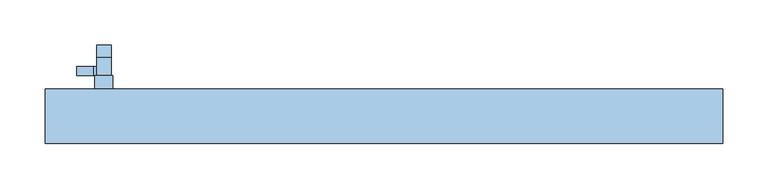
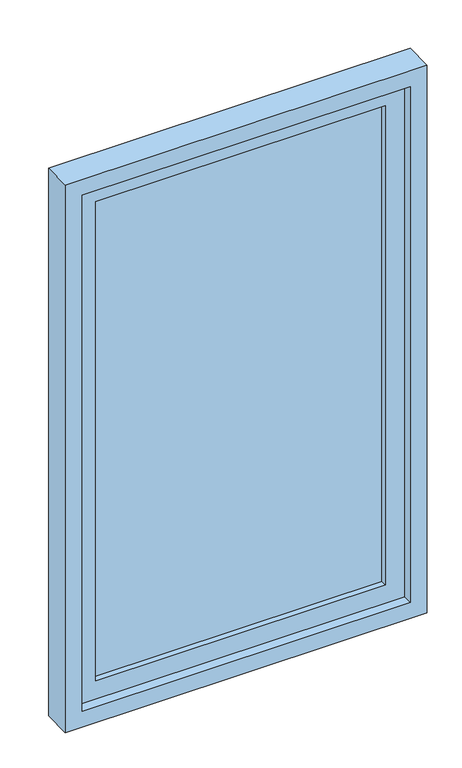
"""IFC4 building model written with IfcOpenShell, lengths in millimetres: window geometry, Inclinar e virar janela - 1 Painel : Inclinar e virar janela - 1 Painel 0,75m."""

from ifc_helpers import new_model, si_unit, point, frame, frame_2d, origin, place, context, project, spatial, polyline, circle_curve, trimmed, segment, composite_curve, outline, extrude, source, transform, mapped, element, save


def window_521f4ff6(model_context):
    return source(origin(), model_context, "Body", "SweptSolid", [
        extrude(outline(composite_curve([segment(polyline([(95.0, 1259.0), (85.0, 1259.0), (85.0, 1277.0), (105.0, 1277.0)]), True, "CONTINUOUS"), segment(trimmed(circle_curve(frame_2d((105.0, 1263.0)), 14.0), [point((105.0, 1277.0))], [point((119.0, 1263.0))], False, "CARTESIAN"), True, "CONTINUOUS"), segment(polyline([(119.0, 1263.0), (119.0, 1120.0), (114.0, 1120.0), (106.9888756, 1235.3294081)]), True, "CONTINUOUS"), segment(trimmed(circle_curve(frame_2d((100.9630874, 1234.9630874)), 6.0369126), [point((106.9888756, 1235.3294081))], [point((100.9630874, 1241.0))], True, "CARTESIAN"), True, "CONTINUOUS"), segment(polyline([(100.9630874, 1241.0), (95.0, 1241.0), (95.0, 1259.0)]), True, "CONTINUOUS")], self_intersect=False)), frame((-318.0, 0.0, 0.0), z_axis=(1.0, 0.0, 0.0), x_axis=(0.0, 1.0, 0.0)), (0.0, 0.0, 1.0), 16.0),
        extrude(outline(polyline([(1259.0, -302.0), (1259.0, -321.9864015), (1257.0348924, -340.0), (1243.0157191, -340.0), (1241.0, -321.9864015), (1241.0, -302.0), (1259.0, -302.0)])), frame((0.0, 85.0, 0.0), z_axis=(0.0, 1.0, 0.0), x_axis=(0.0, 0.0, 1.0)), (0.0, 0.0, 1.0), 10.0),
        extrude(outline(polyline([(-320.0, 85.0), (-300.0, 85.0), (-300.0, 70.0), (-320.0, 70.0), (-320.0, 85.0)])), frame((0.0, 0.0, 1218.0), z_axis=(0.0, 0.0, 1.0), x_axis=(1.0, 0.0, 0.0)), (0.0, 0.0, 1.0), 64.0),
        extrude(outline(polyline([(300.0, 43.0), (-300.0, 43.0), (-300.0, 57.0), (300.0, 57.0), (300.0, 43.0)])), frame((0.0, 0.0, 725.0), z_axis=(0.0, 0.0, 1.0), x_axis=(1.0, 0.0, 0.0)), (0.0, 0.0, 1.0), 1050.0),
        extrude(outline(polyline([(1815.0, -340.0), (685.0, -340.0), (685.0, 340.0), (1815.0, 340.0), (1815.0, -340.0)]), holes=[polyline([(725.0, -300.0), (1775.0, -300.0), (1775.0, 300.0), (725.0, 300.0), (725.0, -300.0)])]), frame((0.0, 30.0, 0.0), z_axis=(0.0, 1.0, 0.0), x_axis=(0.0, 0.0, 1.0)), (0.0, 0.0, 1.0), 40.0),
        extrude(outline(polyline([(1850.0, -375.0), (650.0, -375.0), (650.0, 375.0), (1850.0, 375.0), (1850.0, -375.0)]), holes=[polyline([(685.0, -340.0), (1815.0, -340.0), (1815.0, 340.0), (685.0, 340.0), (685.0, -340.0)])]), frame((0.0, 10.0, 0.0), z_axis=(0.0, 1.0, 0.0), x_axis=(0.0, 0.0, 1.0)), (0.0, 0.0, 1.0), 60.0),
    ])


if __name__ == "__main__":
    model = new_model("IFC4")
    model_context = context("Model", 3, world=origin())
    ifc_project = project(units=[si_unit("LENGTHUNIT", "METRE", prefix="MILLI")], contexts=[model_context])
    site = spatial("IfcSite", under=ifc_project)
    building = spatial("IfcBuilding", under=site)
    placement = place(None, origin())
    window_shape = window_521f4ff6(model_context)
    element("IfcWindow", 1, ObjectType="Inclinar e virar janela - 1 Painel : Inclinar e virar janela - 1 Painel 0,75m", at=placement, inside=building, context=model_context, shape_type="MappedRepresentation", body=[
        mapped(window_shape, transform((0.0, 0.0, 0.0), x_axis=(1.0, 0.0, 0.0), y_axis=(0.0, 1.0, 0.0), z_axis=(0.0, 0.0, 1.0))),
    ])
    save(model, "model.ifc")

# Revit data of these elements
# Type "Inclinar e virar janela - 1 Painel : Inclinar e virar janela - 1 Painel 0,75m"
#   Type Mark = "EF30"
#   Construction Type Id = "SGL"
#   Analytic Construction = "Janelas grandes envidraçadas únicas"
#   W1 = 0.680 m
#   Visual Light Transmittance = 0.9
#   Solar Heat Gain Coefficient = 0.86
#   Rough Width = 0.750 m
#   Rough Height = 1.200 m
#   Largura da moldura do painel = 0.040 m
#   Espessura da moldura do painel = 0.040 m
#   Height = 1.200 m
#   Heat Transfer Coefficient (U) = 5.5617 W/(m²·K)
#   H1 = 1.130 m
#   Largura da estrutura = 0.035 m
#   Espessura da moldura = 0.060 m
#   Altura-padrão do peitoril = 0.650 m
#   Width = 0.750 m
#   Define Thermal Properties by = 1
#   Material do puxador = none
#   Vidro = none
#   Material da moldura = none
#   Wall Closure = (empty or 0)
# Element 1 (IfcWindow, "Inclinar e virar janela - 1 Painel : Inclinar e virar janela - 1 Painel 0,75m")
#   Materials on its faces: "Glass"
# Materials
#   "Glass": class "Glass", colour RGB 0 128 192, transparency 0.75, Description = "Soda Lime Glass", Cost = 0
